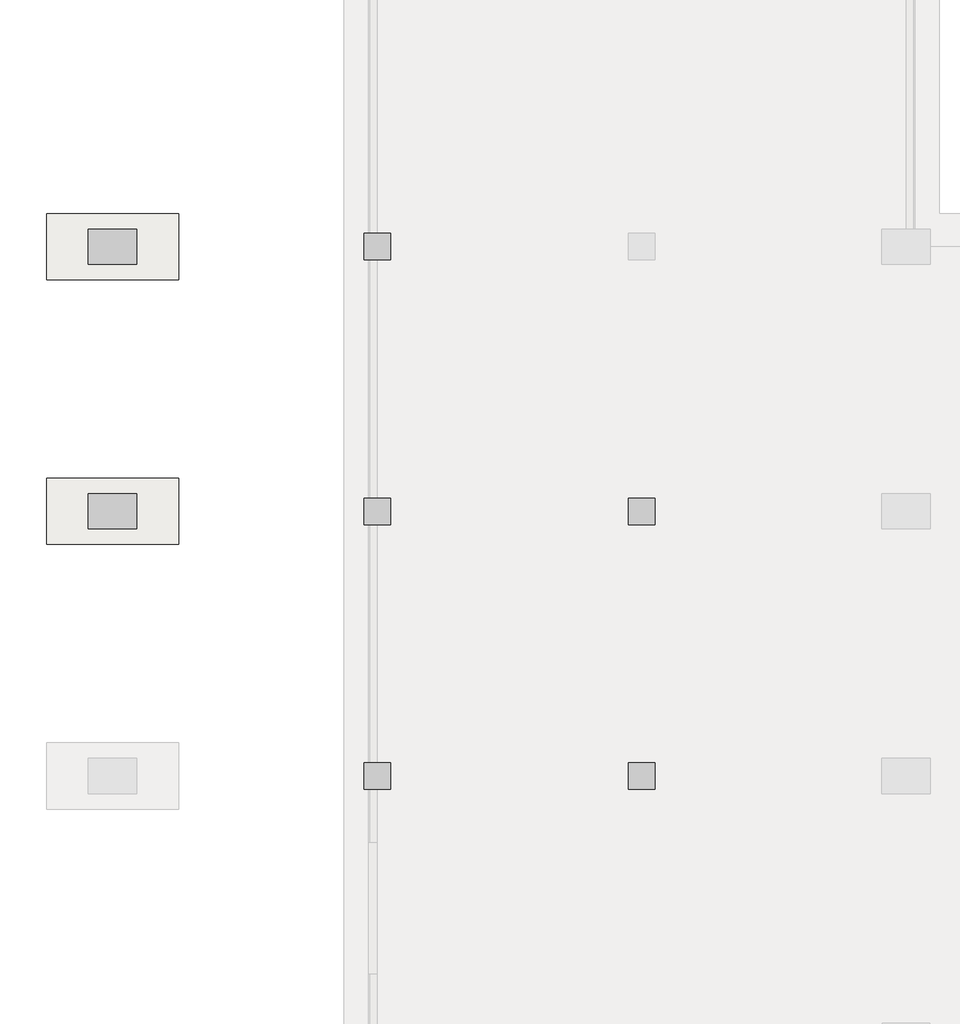
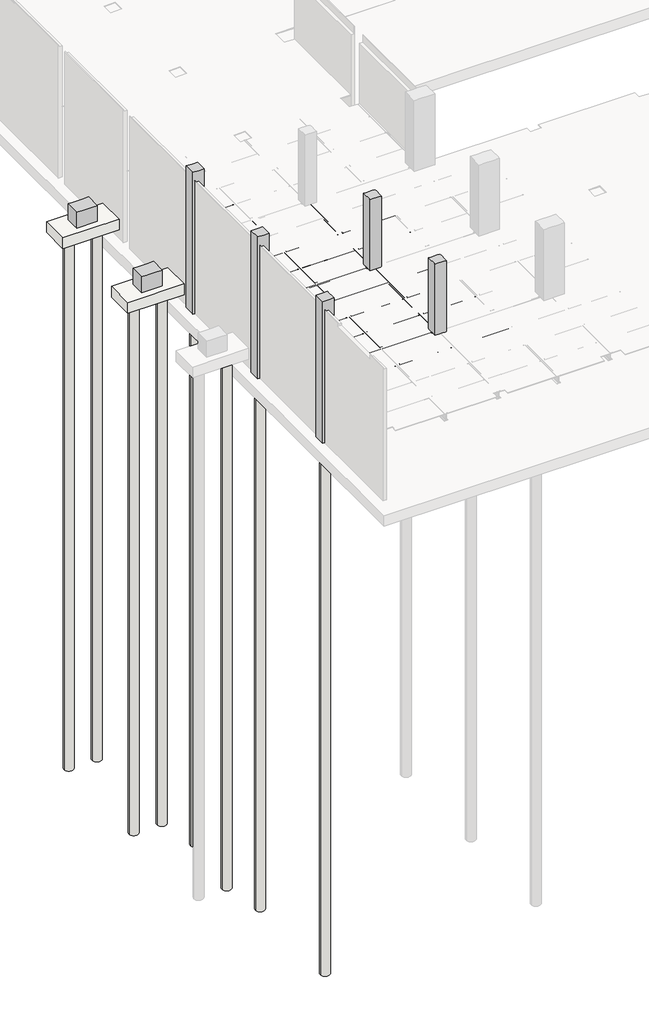
# Not in any storey, part 2 of 16: 26 beams, 10 slabs, 7 columns.
"""IFC4 building model written with IfcOpenShell, lengths in millimetres."""

from ifc_helpers import new_model, si_unit, point, frame, frame_2d, origin, place, context, project, spatial, polyline, circle_curve, trimmed, segment, composite_curve, outline, extrude, faceted_brep, element, save

model = new_model("IFC4")

# Units and contexts
model_context = context("Model", 3, world=origin())
ifc_project = project(units=[si_unit("LENGTHUNIT", "METRE", prefix="MILLI")], contexts=[model_context])

# Site, building
site = spatial("IfcSite", under=ifc_project)
building = spatial("IfcBuilding", under=site)

# Beams
placement = place(None, origin())
element("IfcBeam", 1, ObjectType="Steel Framing_H_KS : H_SB_AR_S02_H-400x200x8x13_BSG1", at=placement, inside=building, context=model_context, shape_type="SweptSolid", body=[
    extrude(outline(composite_curve([segment(polyline([(-47900.0, -4187.0381366), (-47900.0, -4200.0381366), (-48100.0, -4200.0381366), (-48100.0, -4187.0381366), (-48020.0, -4187.0381366)]), True, "CONTINUOUS"), segment(trimmed(circle_curve(frame_2d((-48020.0, -4171.0381366)), 16.0), [point((-48020.0, -4187.0381366))], [point((-48004.0, -4171.0381366))], True, "CARTESIAN"), True, "CONTINUOUS"), segment(polyline([(-48004.0, -4171.0381366), (-48004.0, -3829.0381366)]), True, "CONTINUOUS"), segment(trimmed(circle_curve(frame_2d((-48020.0, -3829.0381366)), 16.0), [point((-48004.0, -3829.0381366))], [point((-48020.0, -3813.0381366))], True, "CARTESIAN"), True, "CONTINUOUS"), segment(polyline([(-48020.0, -3813.0381366), (-48100.0, -3813.0381366), (-48100.0, -3800.0381366), (-47900.0, -3800.0381366), (-47900.0, -3813.0381366), (-47980.0, -3813.0381366)]), True, "CONTINUOUS"), segment(trimmed(circle_curve(frame_2d((-47980.0, -3829.0381366)), 16.0), [point((-47980.0, -3813.0381366))], [point((-47996.0, -3829.0381366))], True, "CARTESIAN"), True, "CONTINUOUS"), segment(polyline([(-47996.0, -3829.0381366), (-47996.0, -4171.0381366)]), True, "CONTINUOUS"), segment(trimmed(circle_curve(frame_2d((-47980.0, -4171.0381366)), 16.0), [point((-47996.0, -4171.0381366))], [point((-47980.0, -4187.0381366))], True, "CARTESIAN"), True, "CONTINUOUS"), segment(polyline([(-47980.0, -4187.0381366), (-47900.0, -4187.0381366)]), True, "CONTINUOUS")], self_intersect=False)), frame((24312.7, 0.0, 0.0), z_axis=(1.0, 0.0, 0.0), x_axis=(0.0, 1.0, 0.0)), (0.0, 0.0, 1.0), 5374.6),
])
element("IfcBeam", 2, ObjectType="Steel Framing_H_KS : H_SB_AR_S02_H-400x200x8x13_BSG2", at=placement, inside=building, context=model_context, shape_type="SweptSolid", body=[
    extrude(outline(composite_curve([segment(polyline([(-4187.0381366, 29900.0), (-4200.0381366, 29900.0), (-4200.0381366, 30100.0), (-4187.0381366, 30100.0), (-4187.0381366, 30020.0)]), True, "CONTINUOUS"), segment(trimmed(circle_curve(frame_2d((-4171.0381366, 30020.0)), 16.0), [point((-4187.0381366, 30020.0))], [point((-4171.0381366, 30004.0))], True, "CARTESIAN"), True, "CONTINUOUS"), segment(polyline([(-4171.0381366, 30004.0), (-3829.0381366, 30004.0)]), True, "CONTINUOUS"), segment(trimmed(circle_curve(frame_2d((-3829.0381366, 30020.0)), 16.0), [point((-3829.0381366, 30004.0))], [point((-3813.0381366, 30020.0))], True, "CARTESIAN"), True, "CONTINUOUS"), segment(polyline([(-3813.0381366, 30020.0), (-3813.0381366, 30100.0), (-3800.0381366, 30100.0), (-3800.0381366, 29900.0), (-3813.0381366, 29900.0), (-3813.0381366, 29980.0)]), True, "CONTINUOUS"), segment(trimmed(circle_curve(frame_2d((-3829.0381366, 29980.0)), 16.0), [point((-3813.0381366, 29980.0))], [point((-3829.0381366, 29996.0))], True, "CARTESIAN"), True, "CONTINUOUS"), segment(polyline([(-3829.0381366, 29996.0), (-4171.0381366, 29996.0)]), True, "CONTINUOUS"), segment(trimmed(circle_curve(frame_2d((-4171.0381366, 29980.0)), 16.0), [point((-4171.0381366, 29996.0))], [point((-4187.0381366, 29980.0))], True, "CARTESIAN"), True, "CONTINUOUS"), segment(polyline([(-4187.0381366, 29980.0), (-4187.0381366, 29900.0)]), True, "CONTINUOUS")], self_intersect=False)), frame((0.0, -47687.3, 0.0), z_axis=(0.0, 1.0, 0.0), x_axis=(0.0, 0.0, 1.0)), (0.0, 0.0, 1.0), 5374.6),
])
element("IfcBeam", 3, ObjectType="Steel Framing_H_KS : H_SB_AR_S02_H-400x200x8x13_BSB1", at=placement, inside=building, context=model_context, shape_type="SweptSolid", body=[
    extrude(outline(composite_curve([segment(polyline([(-4187.0381366, 26900.0), (-4200.0381366, 26900.0), (-4200.0381366, 27100.0), (-4187.0381366, 27100.0), (-4187.0381366, 27020.0)]), True, "CONTINUOUS"), segment(trimmed(circle_curve(frame_2d((-4171.0381366, 27020.0)), 16.0), [point((-4187.0381366, 27020.0))], [point((-4171.0381366, 27004.0))], True, "CARTESIAN"), True, "CONTINUOUS"), segment(polyline([(-4171.0381366, 27004.0), (-3829.0381366, 27004.0)]), True, "CONTINUOUS"), segment(trimmed(circle_curve(frame_2d((-3829.0381366, 27020.0)), 16.0), [point((-3829.0381366, 27004.0))], [point((-3813.0381366, 27020.0))], True, "CARTESIAN"), True, "CONTINUOUS"), segment(polyline([(-3813.0381366, 27020.0), (-3813.0381366, 27100.0), (-3800.0381366, 27100.0), (-3800.0381366, 26900.0), (-3813.0381366, 26900.0), (-3813.0381366, 26980.0)]), True, "CONTINUOUS"), segment(trimmed(circle_curve(frame_2d((-3829.0381366, 26980.0)), 16.0), [point((-3813.0381366, 26980.0))], [point((-3829.0381366, 26996.0))], True, "CARTESIAN"), True, "CONTINUOUS"), segment(polyline([(-3829.0381366, 26996.0), (-4171.0381366, 26996.0)]), True, "CONTINUOUS"), segment(trimmed(circle_curve(frame_2d((-4171.0381366, 26980.0)), 16.0), [point((-4171.0381366, 26996.0))], [point((-4187.0381366, 26980.0))], True, "CARTESIAN"), True, "CONTINUOUS"), segment(polyline([(-4187.0381366, 26980.0), (-4187.0381366, 26900.0)]), True, "CONTINUOUS")], self_intersect=False)), frame((0.0, -47887.3, 0.0), z_axis=(0.0, 1.0, 0.0), x_axis=(0.0, 0.0, 1.0)), (0.0, 0.0, 1.0), 5774.6),
])
element("IfcBeam", 4, ObjectType="Steel Framing_C_KS : H_SB_AR_S02_C-150x75x6.5x10_J1", at=placement, inside=building, context=model_context, shape_type="SweptSolid", body=[
    extrude(outline(composite_curve([segment(polyline([(-44977.2, -3800.0381366), (-44977.2, -3950.0381366), (-45052.2, -3950.0381366)]), True, "CONTINUOUS"), segment(trimmed(circle_curve(frame_2d((-45042.2, -3950.0381366)), 10.0), [point((-45052.2, -3950.0381366))], [point((-45042.2, -3940.0381366))], False, "CARTESIAN"), True, "CONTINUOUS"), segment(polyline([(-45042.2, -3940.0381366), (-44983.7, -3930.7726469), (-44983.7, -3819.3036264), (-45042.2, -3810.0381366)]), True, "CONTINUOUS"), segment(trimmed(circle_curve(frame_2d((-45042.2, -3800.0381366)), 10.0), [point((-45042.2, -3810.0381366))], [point((-45052.2, -3800.0381366))], False, "CARTESIAN"), True, "CONTINUOUS"), segment(polyline([(-45052.2, -3800.0381366), (-44977.2, -3800.0381366)]), True, "CONTINUOUS")], self_intersect=False)), frame((24000.0, 0.0, 0.0), z_axis=(1.0, 0.0, 0.0), x_axis=(0.0, 1.0, 0.0)), (0.0, 0.0, 1.0), 2887.3),
])
element("IfcBeam", 5, ObjectType="Steel Framing_C_KS : H_SB_AR_S02_C-150x75x6.5x10_J1", at=placement, inside=building, context=model_context, shape_type="SweptSolid", body=[
    extrude(outline(composite_curve([segment(polyline([(-46477.2, -3800.0381366), (-46477.2, -3950.0381366), (-46552.2, -3950.0381366)]), True, "CONTINUOUS"), segment(trimmed(circle_curve(frame_2d((-46542.2, -3950.0381366)), 10.0), [point((-46552.2, -3950.0381366))], [point((-46542.2, -3940.0381366))], False, "CARTESIAN"), True, "CONTINUOUS"), segment(polyline([(-46542.2, -3940.0381366), (-46483.7, -3930.7726469), (-46483.7, -3819.3036264), (-46542.2, -3810.0381366)]), True, "CONTINUOUS"), segment(trimmed(circle_curve(frame_2d((-46542.2, -3800.0381366)), 10.0), [point((-46542.2, -3810.0381366))], [point((-46552.2, -3800.0381366))], False, "CARTESIAN"), True, "CONTINUOUS"), segment(polyline([(-46552.2, -3800.0381366), (-46477.2, -3800.0381366)]), True, "CONTINUOUS")], self_intersect=False)), frame((24000.0, 0.0, 0.0), z_axis=(1.0, 0.0, 0.0), x_axis=(0.0, 1.0, 0.0)), (0.0, 0.0, 1.0), 2887.3),
])
element("IfcBeam", 6, ObjectType="Steel Framing_C_KS : H_SB_AR_S02_C-150x75x6.5x10_J1", at=placement, inside=building, context=model_context, shape_type="SweptSolid", body=[
    extrude(outline(composite_curve([segment(polyline([(-43477.2, -3800.0381366), (-43477.2, -3950.0381366), (-43552.2, -3950.0381366)]), True, "CONTINUOUS"), segment(trimmed(circle_curve(frame_2d((-43542.2, -3950.0381366)), 10.0), [point((-43552.2, -3950.0381366))], [point((-43542.2, -3940.0381366))], False, "CARTESIAN"), True, "CONTINUOUS"), segment(polyline([(-43542.2, -3940.0381366), (-43483.7, -3930.7726469), (-43483.7, -3819.3036264), (-43542.2, -3810.0381366)]), True, "CONTINUOUS"), segment(trimmed(circle_curve(frame_2d((-43542.2, -3800.0381366)), 10.0), [point((-43542.2, -3810.0381366))], [point((-43552.2, -3800.0381366))], False, "CARTESIAN"), True, "CONTINUOUS"), segment(polyline([(-43552.2, -3800.0381366), (-43477.2, -3800.0381366)]), True, "CONTINUOUS")], self_intersect=False)), frame((24000.0, 0.0, 0.0), z_axis=(1.0, 0.0, 0.0), x_axis=(0.0, 1.0, 0.0)), (0.0, 0.0, 1.0), 2887.3),
])
element("IfcBeam", 7, ObjectType="Steel Framing_C_KS : H_SB_AR_S02_C-150x75x6.5x10_J1", at=placement, inside=building, context=model_context, shape_type="SweptSolid", body=[
    extrude(outline(composite_curve([segment(polyline([(-44977.2, -3800.0381366), (-44977.2, -3950.0381366), (-45052.2, -3950.0381366)]), True, "CONTINUOUS"), segment(trimmed(circle_curve(frame_2d((-45042.2, -3950.0381366)), 10.0), [point((-45052.2, -3950.0381366))], [point((-45042.2, -3940.0381366))], False, "CARTESIAN"), True, "CONTINUOUS"), segment(polyline([(-45042.2, -3940.0381366), (-44983.7, -3930.7726469), (-44983.7, -3819.3036264), (-45042.2, -3810.0381366)]), True, "CONTINUOUS"), segment(trimmed(circle_curve(frame_2d((-45042.2, -3800.0381366)), 10.0), [point((-45042.2, -3810.0381366))], [point((-45052.2, -3800.0381366))], False, "CARTESIAN"), True, "CONTINUOUS"), segment(polyline([(-45052.2, -3800.0381366), (-44977.2, -3800.0381366)]), True, "CONTINUOUS")], self_intersect=False)), frame((27112.7, 0.0, 0.0), z_axis=(1.0, 0.0, 0.0), x_axis=(0.0, 1.0, 0.0)), (0.0, 0.0, 1.0), 2774.6),
])
element("IfcBeam", 8, ObjectType="Steel Framing_C_KS : H_SB_AR_S02_C-150x75x6.5x10_J1", at=placement, inside=building, context=model_context, shape_type="SweptSolid", body=[
    extrude(outline(composite_curve([segment(polyline([(-46477.2, -3800.0381366), (-46477.2, -3950.0381366), (-46552.2, -3950.0381366)]), True, "CONTINUOUS"), segment(trimmed(circle_curve(frame_2d((-46542.2, -3950.0381366)), 10.0), [point((-46552.2, -3950.0381366))], [point((-46542.2, -3940.0381366))], False, "CARTESIAN"), True, "CONTINUOUS"), segment(polyline([(-46542.2, -3940.0381366), (-46483.7, -3930.7726469), (-46483.7, -3819.3036264), (-46542.2, -3810.0381366)]), True, "CONTINUOUS"), segment(trimmed(circle_curve(frame_2d((-46542.2, -3800.0381366)), 10.0), [point((-46542.2, -3810.0381366))], [point((-46552.2, -3800.0381366))], False, "CARTESIAN"), True, "CONTINUOUS"), segment(polyline([(-46552.2, -3800.0381366), (-46477.2, -3800.0381366)]), True, "CONTINUOUS")], self_intersect=False)), frame((27112.7, 0.0, 0.0), z_axis=(1.0, 0.0, 0.0), x_axis=(0.0, 1.0, 0.0)), (0.0, 0.0, 1.0), 2774.6),
])
element("IfcBeam", 9, ObjectType="Steel Framing_C_KS : H_SB_AR_S02_C-150x75x6.5x10_J1", at=placement, inside=building, context=model_context, shape_type="SweptSolid", body=[
    extrude(outline(composite_curve([segment(polyline([(-44977.2, -3800.0381366), (-44977.2, -3950.0381366), (-45052.2, -3950.0381366)]), True, "CONTINUOUS"), segment(trimmed(circle_curve(frame_2d((-45042.2, -3950.0381366)), 10.0), [point((-45052.2, -3950.0381366))], [point((-45042.2, -3940.0381366))], False, "CARTESIAN"), True, "CONTINUOUS"), segment(polyline([(-45042.2, -3940.0381366), (-44983.7, -3930.7726469), (-44983.7, -3819.3036264), (-45042.2, -3810.0381366)]), True, "CONTINUOUS"), segment(trimmed(circle_curve(frame_2d((-45042.2, -3800.0381366)), 10.0), [point((-45042.2, -3810.0381366))], [point((-45052.2, -3800.0381366))], False, "CARTESIAN"), True, "CONTINUOUS"), segment(polyline([(-45052.2, -3800.0381366), (-44977.2, -3800.0381366)]), True, "CONTINUOUS")], self_intersect=False)), frame((30112.7, 0.0, 0.0), z_axis=(1.0, 0.0, 0.0), x_axis=(0.0, 1.0, 0.0)), (0.0, 0.0, 1.0), 2774.6),
])
element("IfcBeam", 10, ObjectType="Steel Framing_C_KS : H_SB_AR_S02_C-150x75x6.5x10_J1", at=placement, inside=building, context=model_context, shape_type="SweptSolid", body=[
    extrude(outline(composite_curve([segment(polyline([(-46477.2, -3800.0381366), (-46477.2, -3950.0381366), (-46552.2, -3950.0381366)]), True, "CONTINUOUS"), segment(trimmed(circle_curve(frame_2d((-46542.2, -3950.0381366)), 10.0), [point((-46552.2, -3950.0381366))], [point((-46542.2, -3940.0381366))], False, "CARTESIAN"), True, "CONTINUOUS"), segment(polyline([(-46542.2, -3940.0381366), (-46483.7, -3930.7726469), (-46483.7, -3819.3036264), (-46542.2, -3810.0381366)]), True, "CONTINUOUS"), segment(trimmed(circle_curve(frame_2d((-46542.2, -3800.0381366)), 10.0), [point((-46542.2, -3810.0381366))], [point((-46552.2, -3800.0381366))], False, "CARTESIAN"), True, "CONTINUOUS"), segment(polyline([(-46552.2, -3800.0381366), (-46477.2, -3800.0381366)]), True, "CONTINUOUS")], self_intersect=False)), frame((30112.7, 0.0, 0.0), z_axis=(1.0, 0.0, 0.0), x_axis=(0.0, 1.0, 0.0)), (0.0, 0.0, 1.0), 2774.6),
])
element("IfcBeam", 11, ObjectType="Steel Framing_H_KS : H_SB_AR_S02_H-400x200x8x13_BSG1", at=placement, inside=building, context=model_context, shape_type="SweptSolid", body=[
    extrude(outline(composite_curve([segment(polyline([(-53900.0, -4187.0381366), (-53900.0, -4200.0381366), (-54100.0, -4200.0381366), (-54100.0, -4187.0381366), (-54020.0, -4187.0381366)]), True, "CONTINUOUS"), segment(trimmed(circle_curve(frame_2d((-54020.0, -4171.0381366)), 16.0), [point((-54020.0, -4187.0381366))], [point((-54004.0, -4171.0381366))], True, "CARTESIAN"), True, "CONTINUOUS"), segment(polyline([(-54004.0, -4171.0381366), (-54004.0, -3829.0381366)]), True, "CONTINUOUS"), segment(trimmed(circle_curve(frame_2d((-54020.0, -3829.0381366)), 16.0), [point((-54004.0, -3829.0381366))], [point((-54020.0, -3813.0381366))], True, "CARTESIAN"), True, "CONTINUOUS"), segment(polyline([(-54020.0, -3813.0381366), (-54100.0, -3813.0381366), (-54100.0, -3800.0381366), (-53900.0, -3800.0381366), (-53900.0, -3813.0381366), (-53980.0, -3813.0381366)]), True, "CONTINUOUS"), segment(trimmed(circle_curve(frame_2d((-53980.0, -3829.0381366)), 16.0), [point((-53980.0, -3813.0381366))], [point((-53996.0, -3829.0381366))], True, "CARTESIAN"), True, "CONTINUOUS"), segment(polyline([(-53996.0, -3829.0381366), (-53996.0, -4171.0381366)]), True, "CONTINUOUS"), segment(trimmed(circle_curve(frame_2d((-53980.0, -4171.0381366)), 16.0), [point((-53996.0, -4171.0381366))], [point((-53980.0, -4187.0381366))], True, "CARTESIAN"), True, "CONTINUOUS"), segment(polyline([(-53980.0, -4187.0381366), (-53900.0, -4187.0381366)]), True, "CONTINUOUS")], self_intersect=False)), frame((24312.7, 0.0, 0.0), z_axis=(1.0, 0.0, 0.0), x_axis=(0.0, 1.0, 0.0)), (0.0, 0.0, 1.0), 5374.6),
])
element("IfcBeam", 12, ObjectType="Steel Framing_H_KS : H_SB_AR_S02_H-400x200x8x13_BSG2", at=placement, inside=building, context=model_context, shape_type="SweptSolid", body=[
    extrude(outline(composite_curve([segment(polyline([(-4187.0381366, 29900.0), (-4200.0381366, 29900.0), (-4200.0381366, 30100.0), (-4187.0381366, 30100.0), (-4187.0381366, 30020.0)]), True, "CONTINUOUS"), segment(trimmed(circle_curve(frame_2d((-4171.0381366, 30020.0)), 16.0), [point((-4187.0381366, 30020.0))], [point((-4171.0381366, 30004.0))], True, "CARTESIAN"), True, "CONTINUOUS"), segment(polyline([(-4171.0381366, 30004.0), (-3829.0381366, 30004.0)]), True, "CONTINUOUS"), segment(trimmed(circle_curve(frame_2d((-3829.0381366, 30020.0)), 16.0), [point((-3829.0381366, 30004.0))], [point((-3813.0381366, 30020.0))], True, "CARTESIAN"), True, "CONTINUOUS"), segment(polyline([(-3813.0381366, 30020.0), (-3813.0381366, 30100.0), (-3800.0381366, 30100.0), (-3800.0381366, 29900.0), (-3813.0381366, 29900.0), (-3813.0381366, 29980.0)]), True, "CONTINUOUS"), segment(trimmed(circle_curve(frame_2d((-3829.0381366, 29980.0)), 16.0), [point((-3813.0381366, 29980.0))], [point((-3829.0381366, 29996.0))], True, "CARTESIAN"), True, "CONTINUOUS"), segment(polyline([(-3829.0381366, 29996.0), (-4171.0381366, 29996.0)]), True, "CONTINUOUS"), segment(trimmed(circle_curve(frame_2d((-4171.0381366, 29980.0)), 16.0), [point((-4171.0381366, 29996.0))], [point((-4187.0381366, 29980.0))], True, "CARTESIAN"), True, "CONTINUOUS"), segment(polyline([(-4187.0381366, 29980.0), (-4187.0381366, 29900.0)]), True, "CONTINUOUS")], self_intersect=False)), frame((0.0, -53687.3, 0.0), z_axis=(0.0, 1.0, 0.0), x_axis=(0.0, 0.0, 1.0)), (0.0, 0.0, 1.0), 5374.6),
])
element("IfcBeam", 13, ObjectType="Steel Framing_H_KS : H_SB_AR_S02_H-400x200x8x13_BSB1", at=placement, inside=building, context=model_context, shape_type="SweptSolid", body=[
    extrude(outline(composite_curve([segment(polyline([(-4187.0381366, 26900.0), (-4200.0381366, 26900.0), (-4200.0381366, 27100.0), (-4187.0381366, 27100.0), (-4187.0381366, 27020.0)]), True, "CONTINUOUS"), segment(trimmed(circle_curve(frame_2d((-4171.0381366, 27020.0)), 16.0), [point((-4187.0381366, 27020.0))], [point((-4171.0381366, 27004.0))], True, "CARTESIAN"), True, "CONTINUOUS"), segment(polyline([(-4171.0381366, 27004.0), (-3829.0381366, 27004.0)]), True, "CONTINUOUS"), segment(trimmed(circle_curve(frame_2d((-3829.0381366, 27020.0)), 16.0), [point((-3829.0381366, 27004.0))], [point((-3813.0381366, 27020.0))], True, "CARTESIAN"), True, "CONTINUOUS"), segment(polyline([(-3813.0381366, 27020.0), (-3813.0381366, 27100.0), (-3800.0381366, 27100.0), (-3800.0381366, 26900.0), (-3813.0381366, 26900.0), (-3813.0381366, 26980.0)]), True, "CONTINUOUS"), segment(trimmed(circle_curve(frame_2d((-3829.0381366, 26980.0)), 16.0), [point((-3813.0381366, 26980.0))], [point((-3829.0381366, 26996.0))], True, "CARTESIAN"), True, "CONTINUOUS"), segment(polyline([(-3829.0381366, 26996.0), (-4171.0381366, 26996.0)]), True, "CONTINUOUS"), segment(trimmed(circle_curve(frame_2d((-4171.0381366, 26980.0)), 16.0), [point((-4171.0381366, 26996.0))], [point((-4187.0381366, 26980.0))], True, "CARTESIAN"), True, "CONTINUOUS"), segment(polyline([(-4187.0381366, 26980.0), (-4187.0381366, 26900.0)]), True, "CONTINUOUS")], self_intersect=False)), frame((0.0, -53887.3, 0.0), z_axis=(0.0, 1.0, 0.0), x_axis=(0.0, 0.0, 1.0)), (0.0, 0.0, 1.0), 5774.6),
])
element("IfcBeam", 14, ObjectType="Steel Framing_C_KS : H_SB_AR_S02_C-150x75x6.5x10_J1", at=placement, inside=building, context=model_context, shape_type="SweptSolid", body=[
    extrude(outline(composite_curve([segment(polyline([(-50977.2, -3800.0381366), (-50977.2, -3950.0381366), (-51052.2, -3950.0381366)]), True, "CONTINUOUS"), segment(trimmed(circle_curve(frame_2d((-51042.2, -3950.0381366)), 10.0), [point((-51052.2, -3950.0381366))], [point((-51042.2, -3940.0381366))], False, "CARTESIAN"), True, "CONTINUOUS"), segment(polyline([(-51042.2, -3940.0381366), (-50983.7, -3930.7726469), (-50983.7, -3819.3036264), (-51042.2, -3810.0381366)]), True, "CONTINUOUS"), segment(trimmed(circle_curve(frame_2d((-51042.2, -3800.0381366)), 10.0), [point((-51042.2, -3810.0381366))], [point((-51052.2, -3800.0381366))], False, "CARTESIAN"), True, "CONTINUOUS"), segment(polyline([(-51052.2, -3800.0381366), (-50977.2, -3800.0381366)]), True, "CONTINUOUS")], self_intersect=False)), frame((24000.0, 0.0, 0.0), z_axis=(1.0, 0.0, 0.0), x_axis=(0.0, 1.0, 0.0)), (0.0, 0.0, 1.0), 2887.3),
])
element("IfcBeam", 15, ObjectType="Steel Framing_C_KS : H_SB_AR_S02_C-150x75x6.5x10_J1", at=placement, inside=building, context=model_context, shape_type="SweptSolid", body=[
    extrude(outline(composite_curve([segment(polyline([(-52477.2, -3800.0381366), (-52477.2, -3950.0381366), (-52552.2, -3950.0381366)]), True, "CONTINUOUS"), segment(trimmed(circle_curve(frame_2d((-52542.2, -3950.0381366)), 10.0), [point((-52552.2, -3950.0381366))], [point((-52542.2, -3940.0381366))], False, "CARTESIAN"), True, "CONTINUOUS"), segment(polyline([(-52542.2, -3940.0381366), (-52483.7, -3930.7726469), (-52483.7, -3819.3036264), (-52542.2, -3810.0381366)]), True, "CONTINUOUS"), segment(trimmed(circle_curve(frame_2d((-52542.2, -3800.0381366)), 10.0), [point((-52542.2, -3810.0381366))], [point((-52552.2, -3800.0381366))], False, "CARTESIAN"), True, "CONTINUOUS"), segment(polyline([(-52552.2, -3800.0381366), (-52477.2, -3800.0381366)]), True, "CONTINUOUS")], self_intersect=False)), frame((24000.0, 0.0, 0.0), z_axis=(1.0, 0.0, 0.0), x_axis=(0.0, 1.0, 0.0)), (0.0, 0.0, 1.0), 2887.3),
])
element("IfcBeam", 16, ObjectType="Steel Framing_C_KS : H_SB_AR_S02_C-150x75x6.5x10_J1", at=placement, inside=building, context=model_context, shape_type="SweptSolid", body=[
    extrude(outline(composite_curve([segment(polyline([(-49477.2, -3800.0381366), (-49477.2, -3950.0381366), (-49552.2, -3950.0381366)]), True, "CONTINUOUS"), segment(trimmed(circle_curve(frame_2d((-49542.2, -3950.0381366)), 10.0), [point((-49552.2, -3950.0381366))], [point((-49542.2, -3940.0381366))], False, "CARTESIAN"), True, "CONTINUOUS"), segment(polyline([(-49542.2, -3940.0381366), (-49483.7, -3930.7726469), (-49483.7, -3819.3036264), (-49542.2, -3810.0381366)]), True, "CONTINUOUS"), segment(trimmed(circle_curve(frame_2d((-49542.2, -3800.0381366)), 10.0), [point((-49542.2, -3810.0381366))], [point((-49552.2, -3800.0381366))], False, "CARTESIAN"), True, "CONTINUOUS"), segment(polyline([(-49552.2, -3800.0381366), (-49477.2, -3800.0381366)]), True, "CONTINUOUS")], self_intersect=False)), frame((24000.0, 0.0, 0.0), z_axis=(1.0, 0.0, 0.0), x_axis=(0.0, 1.0, 0.0)), (0.0, 0.0, 1.0), 2887.3),
])
element("IfcBeam", 17, ObjectType="Steel Framing_C_KS : H_SB_AR_S02_C-150x75x6.5x10_J1", at=placement, inside=building, context=model_context, shape_type="SweptSolid", body=[
    extrude(outline(composite_curve([segment(polyline([(-50977.2, -3800.0381366), (-50977.2, -3950.0381366), (-51052.2, -3950.0381366)]), True, "CONTINUOUS"), segment(trimmed(circle_curve(frame_2d((-51042.2, -3950.0381366)), 10.0), [point((-51052.2, -3950.0381366))], [point((-51042.2, -3940.0381366))], False, "CARTESIAN"), True, "CONTINUOUS"), segment(polyline([(-51042.2, -3940.0381366), (-50983.7, -3930.7726469), (-50983.7, -3819.3036264), (-51042.2, -3810.0381366)]), True, "CONTINUOUS"), segment(trimmed(circle_curve(frame_2d((-51042.2, -3800.0381366)), 10.0), [point((-51042.2, -3810.0381366))], [point((-51052.2, -3800.0381366))], False, "CARTESIAN"), True, "CONTINUOUS"), segment(polyline([(-51052.2, -3800.0381366), (-50977.2, -3800.0381366)]), True, "CONTINUOUS")], self_intersect=False)), frame((27112.7, 0.0, 0.0), z_axis=(1.0, 0.0, 0.0), x_axis=(0.0, 1.0, 0.0)), (0.0, 0.0, 1.0), 2774.6),
])
element("IfcBeam", 18, ObjectType="Steel Framing_C_KS : H_SB_AR_S02_C-150x75x6.5x10_J1", at=placement, inside=building, context=model_context, shape_type="SweptSolid", body=[
    extrude(outline(composite_curve([segment(polyline([(-52477.2, -3800.0381366), (-52477.2, -3950.0381366), (-52552.2, -3950.0381366)]), True, "CONTINUOUS"), segment(trimmed(circle_curve(frame_2d((-52542.2, -3950.0381366)), 10.0), [point((-52552.2, -3950.0381366))], [point((-52542.2, -3940.0381366))], False, "CARTESIAN"), True, "CONTINUOUS"), segment(polyline([(-52542.2, -3940.0381366), (-52483.7, -3930.7726469), (-52483.7, -3819.3036264), (-52542.2, -3810.0381366)]), True, "CONTINUOUS"), segment(trimmed(circle_curve(frame_2d((-52542.2, -3800.0381366)), 10.0), [point((-52542.2, -3810.0381366))], [point((-52552.2, -3800.0381366))], False, "CARTESIAN"), True, "CONTINUOUS"), segment(polyline([(-52552.2, -3800.0381366), (-52477.2, -3800.0381366)]), True, "CONTINUOUS")], self_intersect=False)), frame((27112.7, 0.0, 0.0), z_axis=(1.0, 0.0, 0.0), x_axis=(0.0, 1.0, 0.0)), (0.0, 0.0, 1.0), 2774.6),
])
element("IfcBeam", 19, ObjectType="Steel Framing_C_KS : H_SB_AR_S02_C-150x75x6.5x10_J1", at=placement, inside=building, context=model_context, shape_type="SweptSolid", body=[
    extrude(outline(composite_curve([segment(polyline([(-49477.2, -3800.0381366), (-49477.2, -3950.0381366), (-49552.2, -3950.0381366)]), True, "CONTINUOUS"), segment(trimmed(circle_curve(frame_2d((-49542.2, -3950.0381366)), 10.0), [point((-49552.2, -3950.0381366))], [point((-49542.2, -3940.0381366))], False, "CARTESIAN"), True, "CONTINUOUS"), segment(polyline([(-49542.2, -3940.0381366), (-49483.7, -3930.7726469), (-49483.7, -3819.3036264), (-49542.2, -3810.0381366)]), True, "CONTINUOUS"), segment(trimmed(circle_curve(frame_2d((-49542.2, -3800.0381366)), 10.0), [point((-49542.2, -3810.0381366))], [point((-49552.2, -3800.0381366))], False, "CARTESIAN"), True, "CONTINUOUS"), segment(polyline([(-49552.2, -3800.0381366), (-49477.2, -3800.0381366)]), True, "CONTINUOUS")], self_intersect=False)), frame((27112.7, 0.0, 0.0), z_axis=(1.0, 0.0, 0.0), x_axis=(0.0, 1.0, 0.0)), (0.0, 0.0, 1.0), 2774.6),
])
element("IfcBeam", 20, ObjectType="Steel Framing_C_KS : H_SB_AR_S02_C-150x75x6.5x10_J1", at=placement, inside=building, context=model_context, shape_type="SweptSolid", body=[
    extrude(outline(composite_curve([segment(polyline([(-50977.2, -3800.0381366), (-50977.2, -3950.0381366), (-51052.2, -3950.0381366)]), True, "CONTINUOUS"), segment(trimmed(circle_curve(frame_2d((-51042.2, -3950.0381366)), 10.0), [point((-51052.2, -3950.0381366))], [point((-51042.2, -3940.0381366))], False, "CARTESIAN"), True, "CONTINUOUS"), segment(polyline([(-51042.2, -3940.0381366), (-50983.7, -3930.7726469), (-50983.7, -3819.3036264), (-51042.2, -3810.0381366)]), True, "CONTINUOUS"), segment(trimmed(circle_curve(frame_2d((-51042.2, -3800.0381366)), 10.0), [point((-51042.2, -3810.0381366))], [point((-51052.2, -3800.0381366))], False, "CARTESIAN"), True, "CONTINUOUS"), segment(polyline([(-51052.2, -3800.0381366), (-50977.2, -3800.0381366)]), True, "CONTINUOUS")], self_intersect=False)), frame((30112.7, 0.0, 0.0), z_axis=(1.0, 0.0, 0.0), x_axis=(0.0, 1.0, 0.0)), (0.0, 0.0, 1.0), 2774.6),
])
element("IfcBeam", 21, ObjectType="Steel Framing_C_KS : H_SB_AR_S02_C-150x75x6.5x10_J1", at=placement, inside=building, context=model_context, shape_type="SweptSolid", body=[
    extrude(outline(composite_curve([segment(polyline([(-52477.2, -3800.0381366), (-52477.2, -3950.0381366), (-52552.2, -3950.0381366)]), True, "CONTINUOUS"), segment(trimmed(circle_curve(frame_2d((-52542.2, -3950.0381366)), 10.0), [point((-52552.2, -3950.0381366))], [point((-52542.2, -3940.0381366))], False, "CARTESIAN"), True, "CONTINUOUS"), segment(polyline([(-52542.2, -3940.0381366), (-52483.7, -3930.7726469), (-52483.7, -3819.3036264), (-52542.2, -3810.0381366)]), True, "CONTINUOUS"), segment(trimmed(circle_curve(frame_2d((-52542.2, -3800.0381366)), 10.0), [point((-52542.2, -3810.0381366))], [point((-52552.2, -3800.0381366))], False, "CARTESIAN"), True, "CONTINUOUS"), segment(polyline([(-52552.2, -3800.0381366), (-52477.2, -3800.0381366)]), True, "CONTINUOUS")], self_intersect=False)), frame((30112.7, 0.0, 0.0), z_axis=(1.0, 0.0, 0.0), x_axis=(0.0, 1.0, 0.0)), (0.0, 0.0, 1.0), 2774.6),
])
element("IfcBeam", 22, ObjectType="Steel Framing_C_KS : H_SB_AR_S02_C-150x75x6.5x10_J1", at=placement, inside=building, context=model_context, shape_type="SweptSolid", body=[
    extrude(outline(composite_curve([segment(polyline([(-49477.2, -3800.0381366), (-49477.2, -3950.0381366), (-49552.2, -3950.0381366)]), True, "CONTINUOUS"), segment(trimmed(circle_curve(frame_2d((-49542.2, -3950.0381366)), 10.0), [point((-49552.2, -3950.0381366))], [point((-49542.2, -3940.0381366))], False, "CARTESIAN"), True, "CONTINUOUS"), segment(polyline([(-49542.2, -3940.0381366), (-49483.7, -3930.7726469), (-49483.7, -3819.3036264), (-49542.2, -3810.0381366)]), True, "CONTINUOUS"), segment(trimmed(circle_curve(frame_2d((-49542.2, -3800.0381366)), 10.0), [point((-49542.2, -3810.0381366))], [point((-49552.2, -3800.0381366))], False, "CARTESIAN"), True, "CONTINUOUS"), segment(polyline([(-49552.2, -3800.0381366), (-49477.2, -3800.0381366)]), True, "CONTINUOUS")], self_intersect=False)), frame((30112.7, 0.0, 0.0), z_axis=(1.0, 0.0, 0.0), x_axis=(0.0, 1.0, 0.0)), (0.0, 0.0, 1.0), 2774.6),
])
element("IfcBeam", 23, ObjectType="Steel Framing_C_KS : H_SB_AR_S02_C-150x75x6.5x10_J1", at=placement, inside=building, context=model_context, shape_type="SweptSolid", body=[
    extrude(outline(composite_curve([segment(polyline([(-55477.2, -3800.0381366), (-55477.2, -3950.0381366), (-55552.2, -3950.0381366)]), True, "CONTINUOUS"), segment(trimmed(circle_curve(frame_2d((-55542.2, -3950.0381366)), 10.0), [point((-55552.2, -3950.0381366))], [point((-55542.2, -3940.0381366))], False, "CARTESIAN"), True, "CONTINUOUS"), segment(polyline([(-55542.2, -3940.0381366), (-55483.7, -3930.7726469), (-55483.7, -3819.3036264), (-55542.2, -3810.0381366)]), True, "CONTINUOUS"), segment(trimmed(circle_curve(frame_2d((-55542.2, -3800.0381366)), 10.0), [point((-55542.2, -3810.0381366))], [point((-55552.2, -3800.0381366))], False, "CARTESIAN"), True, "CONTINUOUS"), segment(polyline([(-55552.2, -3800.0381366), (-55477.2, -3800.0381366)]), True, "CONTINUOUS")], self_intersect=False)), frame((24000.0, 0.0, 0.0), z_axis=(1.0, 0.0, 0.0), x_axis=(0.0, 1.0, 0.0)), (0.0, 0.0, 1.0), 2887.3),
])
element("IfcBeam", 24, ObjectType="Steel Framing_C_KS : H_SB_AR_S02_C-150x75x6.5x10_J1", at=placement, inside=building, context=model_context, shape_type="SweptSolid", body=[
    extrude(outline(composite_curve([segment(polyline([(-55477.2, -3800.0381366), (-55477.2, -3950.0381366), (-55552.2, -3950.0381366)]), True, "CONTINUOUS"), segment(trimmed(circle_curve(frame_2d((-55542.2, -3950.0381366)), 10.0), [point((-55552.2, -3950.0381366))], [point((-55542.2, -3940.0381366))], False, "CARTESIAN"), True, "CONTINUOUS"), segment(polyline([(-55542.2, -3940.0381366), (-55483.7, -3930.7726469), (-55483.7, -3819.3036264), (-55542.2, -3810.0381366)]), True, "CONTINUOUS"), segment(trimmed(circle_curve(frame_2d((-55542.2, -3800.0381366)), 10.0), [point((-55542.2, -3810.0381366))], [point((-55552.2, -3800.0381366))], False, "CARTESIAN"), True, "CONTINUOUS"), segment(polyline([(-55552.2, -3800.0381366), (-55477.2, -3800.0381366)]), True, "CONTINUOUS")], self_intersect=False)), frame((27112.7, 0.0, 0.0), z_axis=(1.0, 0.0, 0.0), x_axis=(0.0, 1.0, 0.0)), (0.0, 0.0, 1.0), 2774.6),
])
element("IfcBeam", 25, ObjectType="Steel Framing_C_KS : H_SB_AR_S02_C-150x75x6.5x10_J1", at=placement, inside=building, context=model_context, shape_type="SweptSolid", body=[
    extrude(outline(composite_curve([segment(polyline([(-55477.2, -3800.0381366), (-55477.2, -3950.0381366), (-55552.2, -3950.0381366)]), True, "CONTINUOUS"), segment(trimmed(circle_curve(frame_2d((-55542.2, -3950.0381366)), 10.0), [point((-55552.2, -3950.0381366))], [point((-55542.2, -3940.0381366))], False, "CARTESIAN"), True, "CONTINUOUS"), segment(polyline([(-55542.2, -3940.0381366), (-55483.7, -3930.7726469), (-55483.7, -3819.3036264), (-55542.2, -3810.0381366)]), True, "CONTINUOUS"), segment(trimmed(circle_curve(frame_2d((-55542.2, -3800.0381366)), 10.0), [point((-55542.2, -3810.0381366))], [point((-55552.2, -3800.0381366))], False, "CARTESIAN"), True, "CONTINUOUS"), segment(polyline([(-55552.2, -3800.0381366), (-55477.2, -3800.0381366)]), True, "CONTINUOUS")], self_intersect=False)), frame((30112.7, 0.0, 0.0), z_axis=(1.0, 0.0, 0.0), x_axis=(0.0, 1.0, 0.0)), (0.0, 0.0, 1.0), 2774.6),
])
element("IfcBeam", 26, ObjectType="Steel Framing_C_KS : H_SB_AR_S02_C-150x75x6.5x10_J1", at=placement, inside=building, context=model_context, shape_type="SweptSolid", body=[
    extrude(outline(composite_curve([segment(polyline([(-40477.2, -3800.0381366), (-40477.2, -3950.0381366), (-40552.2, -3950.0381366)]), True, "CONTINUOUS"), segment(trimmed(circle_curve(frame_2d((-40542.2, -3950.0381366)), 10.0), [point((-40552.2, -3950.0381366))], [point((-40542.2, -3940.0381366))], False, "CARTESIAN"), True, "CONTINUOUS"), segment(polyline([(-40542.2, -3940.0381366), (-40483.7, -3930.7726469), (-40483.7, -3819.3036264), (-40542.2, -3810.0381366)]), True, "CONTINUOUS"), segment(trimmed(circle_curve(frame_2d((-40542.2, -3800.0381366)), 10.0), [point((-40542.2, -3810.0381366))], [point((-40552.2, -3800.0381366))], False, "CARTESIAN"), True, "CONTINUOUS"), segment(polyline([(-40552.2, -3800.0381366), (-40477.2, -3800.0381366)]), True, "CONTINUOUS")], self_intersect=False)), frame((24000.0, 0.0, 0.0), z_axis=(1.0, 0.0, 0.0), x_axis=(0.0, 1.0, 0.0)), (0.0, 0.0, 1.0), 2887.3),
])

# Columns
element("IfcColumn", 27, ObjectType="RC_Column_Rectangular : H_SC_AR_S15_UG PED_Bit_800x1100_PD1", at=placement, inside=building, context=model_context, shape_type="Brep", body=[
    faceted_brep([(17450.0, -41600.0, -700.0381366), (18550.0, -41600.0, -700.0381366), (18550.0, -42400.0, -700.0381366), (17450.0, -42400.0, -700.0381366), (17450.0, -41600.0, 199.9618634), (17800.0, -41600.0, 199.9618634), (18200.0, -41600.0, 199.9618634), (18550.0, -41600.0, 199.9618634), (18550.0, -41600.0, -0.0381366), (18550.0, -42400.0, 199.9618634), (18550.0, -42400.0, -0.0381366), (18200.0, -42400.0, 199.9618634), (17800.0, -42400.0, 199.9618634), (17450.0, -42400.0, 199.9618634)], [[[0, 1, 2, 3]], [[4, 5, 6, 7, 8, 1, 0]], [[7, 9, 10, 2, 1, 8]], [[9, 11, 12, 13, 3, 2, 10]], [[13, 4, 0, 3]], [[4, 13, 12, 11, 9, 7, 6, 5]]]),
])
element("IfcColumn", 28, ObjectType="RC_Column_Rectangular : H_SC_AR_S15_UG PED_Bit_800x1100_PD1", at=placement, inside=building, context=model_context, shape_type="Brep", body=[
    faceted_brep([(17450.0, -47600.0, -700.0381366), (18550.0, -47600.0, -700.0381366), (18550.0, -48400.0, -700.0381366), (17450.0, -48400.0, -700.0381366), (17450.0, -47600.0, 199.9618634), (17800.0, -47600.0, 199.9618634), (18200.0, -47600.0, 199.9618634), (18550.0, -47600.0, 199.9618634), (18550.0, -47600.0, -0.0381366), (18550.0, -48400.0, 199.9618634), (18550.0, -48400.0, -0.0381366), (18200.0, -48400.0, 199.9618634), (17800.0, -48400.0, 199.9618634), (17450.0, -48400.0, 199.9618634)], [[[0, 1, 2, 3]], [[4, 5, 6, 7, 8, 1, 0]], [[7, 9, 10, 2, 1, 8]], [[9, 11, 12, 13, 3, 2, 10]], [[13, 4, 0, 3]], [[4, 13, 12, 11, 9, 7, 6, 5]]]),
])
element("IfcColumn", 29, ObjectType="RC_Column_Rectangular : H_SC_AR_S15_UG PED_Bit_600x600_BC1", at=placement, inside=building, context=model_context, shape_type="Brep", body=[
    faceted_brep([(24300.0, -41700.0, -7800.0381366), (24300.0, -42300.0, -7800.0381366), (24000.0, -42300.0, -7800.0381366), (23800.0, -42300.0, -7800.0381366), (23700.0, -42300.0, -7800.0381366), (23700.0, -41700.0, -7800.0381366), (23800.0, -41700.0, -7800.0381366), (24000.0, -41700.0, -7800.0381366), (24300.0, -41700.0, 199.9618634), (24300.0, -41825.0, 199.9618634), (24300.0, -42175.0, 199.9618634), (24300.0, -42300.0, 199.9618634), (24300.0, -42300.0, -0.0381366), (24300.0, -42300.0, -3800.0381366), (24300.0, -42300.0, -3832.0381366), (24300.0, -41700.0, -3832.0381366), (24300.0, -41700.0, -3800.0381366), (24300.0, -41700.0, -0.0381366), (24000.0, -42300.0, 199.9618634), (23700.0, -42300.0, 199.9618634), (23700.0, -42300.0, -0.0381366), (23700.0, -41700.0, 199.9618634), (23700.0, -41700.0, -0.0381366), (24000.0, -41700.0, 199.9618634)], [[[0, 1, 2, 3, 4, 5, 6, 7]], [[8, 9, 10, 11, 12, 13, 14, 1, 0, 15, 16, 17]], [[11, 18, 19, 20, 4, 3, 2, 1, 14, 13, 12]], [[19, 21, 22, 5, 4, 20]], [[21, 23, 8, 17, 16, 15, 0, 7, 6, 5, 22]], [[8, 23, 21, 19, 18, 11, 10, 9]]]),
])
element("IfcColumn", 30, ObjectType="RC_Column_Rectangular : H_SC_AR_S15_UG PED_Bit_600x600_BC1", at=placement, inside=building, context=model_context, shape_type="Brep", body=[
    faceted_brep([(30300.0, -47700.0, -7200.0381366), (30300.0, -48300.0, -7200.0381366), (29700.0, -48300.0, -7200.0381366), (29700.0, -47700.0, -7200.0381366), (30300.0, -47700.0, 199.9618634), (30300.0, -47825.0, 199.9618634), (30300.0, -48175.0, 199.9618634), (30300.0, -48300.0, 199.9618634), (30300.0, -48300.0, 167.9618634), (30300.0, -48300.0, -3800.0381366), (30300.0, -48300.0, -3832.0381366), (30300.0, -47700.0, -3832.0381366), (30300.0, -47700.0, -3800.0381366), (30300.0, -47700.0, 167.9618634), (30175.0, -48300.0, 199.9618634), (29825.0, -48300.0, 199.9618634), (29700.0, -48300.0, 199.9618634), (29700.0, -48300.0, -0.0381366), (29700.0, -48300.0, -3800.0381366), (29700.0, -48300.0, -3832.0381366), (29700.0, -48175.0, 199.9618634), (29700.0, -47825.0, 199.9618634), (29700.0, -47700.0, 199.9618634), (29700.0, -47700.0, -0.0381366), (29700.0, -47700.0, -3800.0381366), (29700.0, -47700.0, -3832.0381366), (29825.0, -47700.0, 199.9618634), (30175.0, -47700.0, 199.9618634)], [[[0, 1, 2, 3]], [[4, 5, 6, 7, 8, 9, 10, 1, 0, 11, 12, 13]], [[7, 14, 15, 16, 17, 18, 19, 2, 1, 10, 9, 8]], [[16, 20, 21, 22, 23, 24, 25, 3, 2, 19, 18, 17]], [[22, 26, 27, 4, 13, 12, 11, 0, 3, 25, 24, 23]], [[4, 27, 26, 22, 21, 20, 16, 15, 14, 7, 6, 5]]]),
])
element("IfcColumn", 31, ObjectType="RC_Column_Rectangular : H_SC_AR_S15_UG PED_Bit_600x600_BC1", at=placement, inside=building, context=model_context, shape_type="Brep", body=[
    faceted_brep([(24300.0, -47700.0, -7800.0381366), (24300.0, -48300.0, -7800.0381366), (24000.0, -48300.0, -7800.0381366), (23800.0, -48300.0, -7800.0381366), (23700.0, -48300.0, -7800.0381366), (23700.0, -47700.0, -7800.0381366), (23800.0, -47700.0, -7800.0381366), (24000.0, -47700.0, -7800.0381366), (24300.0, -47700.0, 199.9618634), (24300.0, -47825.0, 199.9618634), (24300.0, -48175.0, 199.9618634), (24300.0, -48300.0, 199.9618634), (24300.0, -48300.0, -0.0381366), (24300.0, -48300.0, -3800.0381366), (24300.0, -48300.0, -3832.0381366), (24300.0, -47700.0, -3832.0381366), (24300.0, -47700.0, -3800.0381366), (24300.0, -47700.0, -0.0381366), (24000.0, -48300.0, 199.9618634), (23700.0, -48300.0, 199.9618634), (23700.0, -48300.0, -0.0381366), (23700.0, -47700.0, 199.9618634), (23700.0, -47700.0, -0.0381366), (24000.0, -47700.0, 199.9618634)], [[[0, 1, 2, 3, 4, 5, 6, 7]], [[8, 9, 10, 11, 12, 13, 14, 1, 0, 15, 16, 17]], [[11, 18, 19, 20, 4, 3, 2, 1, 14, 13, 12]], [[19, 21, 22, 5, 4, 20]], [[21, 23, 8, 17, 16, 15, 0, 7, 6, 5, 22]], [[8, 23, 21, 19, 18, 11, 10, 9]]]),
])
element("IfcColumn", 32, ObjectType="RC_Column_Rectangular : H_SC_AR_S15_UG PED_Bit_600x600_BC1", at=placement, inside=building, context=model_context, shape_type="Brep", body=[
    faceted_brep([(30300.0, -53700.0, -7200.0381366), (30300.0, -54300.0, -7200.0381366), (29700.0, -54300.0, -7200.0381366), (29700.0, -53700.0, -7200.0381366), (30300.0, -53700.0, 199.9618634), (30300.0, -53825.0, 199.9618634), (30300.0, -54175.0, 199.9618634), (30300.0, -54300.0, 199.9618634), (30300.0, -54300.0, -0.0381366), (30300.0, -54300.0, -3800.0381366), (30300.0, -54300.0, -3832.0381366), (30300.0, -53700.0, -3832.0381366), (30300.0, -53700.0, -3800.0381366), (30300.0, -53700.0, 167.9618634), (30175.0, -54300.0, 199.9618634), (29825.0, -54300.0, 199.9618634), (29700.0, -54300.0, 199.9618634), (29700.0, -54300.0, -0.0381366), (29700.0, -54300.0, -3800.0381366), (29700.0, -54300.0, -3832.0381366), (29700.0, -54175.0, 199.9618634), (29700.0, -53825.0, 199.9618634), (29700.0, -53700.0, 199.9618634), (29700.0, -53700.0, -0.0381366), (29700.0, -53700.0, -3800.0381366), (29700.0, -53700.0, -3832.0381366), (29825.0, -53700.0, 199.9618634), (30175.0, -53700.0, 199.9618634)], [[[0, 1, 2, 3]], [[4, 5, 6, 7, 8, 9, 10, 1, 0, 11, 12, 13]], [[7, 14, 15, 16, 17, 18, 19, 2, 1, 10, 9, 8]], [[16, 20, 21, 22, 23, 24, 25, 3, 2, 19, 18, 17]], [[22, 26, 27, 4, 13, 12, 11, 0, 3, 25, 24, 23]], [[4, 27, 26, 22, 21, 20, 16, 15, 14, 7, 6, 5]]]),
])
element("IfcColumn", 33, ObjectType="RC_Column_Rectangular : H_SC_AR_S15_UG PED_Bit_600x600_BC1", at=placement, inside=building, context=model_context, shape_type="Brep", body=[
    faceted_brep([(24300.0, -53700.0, -7800.0381366), (24300.0, -54300.0, -7800.0381366), (24000.0, -54300.0, -7800.0381366), (23800.0, -54300.0, -7800.0381366), (23700.0, -54300.0, -7800.0381366), (23700.0, -53700.0, -7800.0381366), (23800.0, -53700.0, -7800.0381366), (24000.0, -53700.0, -7800.0381366), (24300.0, -53700.0, 199.9618634), (24300.0, -53825.0, 199.9618634), (24300.0, -54175.0, 199.9618634), (24300.0, -54300.0, 199.9618634), (24300.0, -54300.0, -0.0381366), (24300.0, -54300.0, -3800.0381366), (24300.0, -54300.0, -3832.0381366), (24300.0, -53700.0, -3832.0381366), (24300.0, -53700.0, -3800.0381366), (24300.0, -53700.0, -0.0381366), (24000.0, -54300.0, 199.9618634), (23700.0, -54300.0, 199.9618634), (23700.0, -54300.0, -0.0381366), (23700.0, -53700.0, 199.9618634), (23700.0, -53700.0, -0.0381366), (24000.0, -53700.0, 199.9618634)], [[[0, 1, 2, 3, 4, 5, 6, 7]], [[8, 9, 10, 11, 12, 13, 14, 1, 0, 15, 16, 17]], [[11, 18, 19, 20, 4, 3, 2, 1, 14, 13, 12]], [[19, 21, 22, 5, 4, 20]], [[21, 23, 8, 17, 16, 15, 0, 7, 6, 5, 22]], [[8, 23, 21, 19, 18, 11, 10, 9]]]),
])

# Slabs
element("IfcSlab", 34, ObjectType="Foundation Rectangular (Non-Pile) : H_SF_AR_S18_Shallow Fdn_Bitumen_1500x3000xT600_F1", at=placement, inside=building, context=model_context, shape_type="SweptSolid", body=[
    extrude(outline(polyline([(19500.0, -42750.0), (16500.0, -42750.0), (16500.0, -41250.0), (19500.0, -41250.0), (19500.0, -42750.0)])), frame((0.0, 0.0, -1300.0381366), z_axis=(0.0, 0.0, 1.0), x_axis=(1.0, 0.0, 0.0)), (0.0, 0.0, 1.0), 600.0),
])
element("IfcSlab", 35, ObjectType="Foundation Rectangular (Non-Pile) : H_SF_AR_S18_Shallow Fdn_Bitumen_1500x3000xT600_F1", at=placement, inside=building, context=model_context, shape_type="SweptSolid", body=[
    extrude(outline(polyline([(19500.0, -48750.0), (16500.0, -48750.0), (16500.0, -47250.0), (19500.0, -47250.0), (19500.0, -48750.0)])), frame((0.0, 0.0, -1300.0381366), z_axis=(0.0, 0.0, 1.0), x_axis=(1.0, 0.0, 0.0)), (0.0, 0.0, 1.0), 600.0),
])
element("IfcSlab", 36, ObjectType="PILE : H_SF_AR_S19_PHC Pile_Pre-boring_D500_L30", at=placement, inside=building, context=model_context, shape_type="SweptSolid", body=[
    extrude(outline(composite_curve([segment(trimmed(circle_curve(frame_2d((18750.0, -54000.0)), 250.0), [point((18500.0, -54000.0))], [point((19000.0, -54000.0))], False, "CARTESIAN"), True, "CONTINUOUS"), segment(trimmed(circle_curve(frame_2d((18750.0, -54000.0)), 250.0), [point((19000.0, -54000.0))], [point((18500.0, -54000.0))], False, "CARTESIAN"), True, "CONTINUOUS")], self_intersect=False)), frame((0.0, 0.0, -31300.0381366), z_axis=(0.0, 0.0, 1.0), x_axis=(1.0, 0.0, 0.0)), (0.0, 0.0, 1.0), 30000.0),
])
element("IfcSlab", 37, ObjectType="PILE : H_SF_AR_S19_PHC Pile_Pre-boring_D500_L30", at=placement, inside=building, context=model_context, shape_type="SweptSolid", body=[
    extrude(outline(composite_curve([segment(trimmed(circle_curve(frame_2d((17250.0, -48000.0)), 250.0), [point((17000.0, -48000.0))], [point((17500.0, -48000.0))], False, "CARTESIAN"), True, "CONTINUOUS"), segment(trimmed(circle_curve(frame_2d((17250.0, -48000.0)), 250.0), [point((17500.0, -48000.0))], [point((17000.0, -48000.0))], False, "CARTESIAN"), True, "CONTINUOUS")], self_intersect=False)), frame((0.0, 0.0, -31300.0381366), z_axis=(0.0, 0.0, 1.0), x_axis=(1.0, 0.0, 0.0)), (0.0, 0.0, 1.0), 30000.0),
])
element("IfcSlab", 38, ObjectType="PILE : H_SF_AR_S19_PHC Pile_Pre-boring_D500_L30", at=placement, inside=building, context=model_context, shape_type="SweptSolid", body=[
    extrude(outline(composite_curve([segment(trimmed(circle_curve(frame_2d((18750.0, -48000.0)), 250.0), [point((18500.0, -48000.0))], [point((19000.0, -48000.0))], False, "CARTESIAN"), True, "CONTINUOUS"), segment(trimmed(circle_curve(frame_2d((18750.0, -48000.0)), 250.0), [point((19000.0, -48000.0))], [point((18500.0, -48000.0))], False, "CARTESIAN"), True, "CONTINUOUS")], self_intersect=False)), frame((0.0, 0.0, -31300.0381366), z_axis=(0.0, 0.0, 1.0), x_axis=(1.0, 0.0, 0.0)), (0.0, 0.0, 1.0), 30000.0),
])
element("IfcSlab", 39, ObjectType="PILE : H_SF_AR_S19_PHC Pile_Pre-boring_D500_L30", at=placement, inside=building, context=model_context, shape_type="SweptSolid", body=[
    extrude(outline(composite_curve([segment(trimmed(circle_curve(frame_2d((17250.0, -42000.0)), 250.0), [point((17000.0, -42000.0))], [point((17500.0, -42000.0))], False, "CARTESIAN"), True, "CONTINUOUS"), segment(trimmed(circle_curve(frame_2d((17250.0, -42000.0)), 250.0), [point((17500.0, -42000.0))], [point((17000.0, -42000.0))], False, "CARTESIAN"), True, "CONTINUOUS")], self_intersect=False)), frame((0.0, 0.0, -31300.0381366), z_axis=(0.0, 0.0, 1.0), x_axis=(1.0, 0.0, 0.0)), (0.0, 0.0, 1.0), 30000.0),
])
element("IfcSlab", 40, ObjectType="PILE : H_SF_AR_S19_PHC Pile_Pre-boring_D500_L30", at=placement, inside=building, context=model_context, shape_type="SweptSolid", body=[
    extrude(outline(composite_curve([segment(trimmed(circle_curve(frame_2d((18750.0, -42000.0)), 250.0), [point((18500.0, -42000.0))], [point((19000.0, -42000.0))], False, "CARTESIAN"), True, "CONTINUOUS"), segment(trimmed(circle_curve(frame_2d((18750.0, -42000.0)), 250.0), [point((19000.0, -42000.0))], [point((18500.0, -42000.0))], False, "CARTESIAN"), True, "CONTINUOUS")], self_intersect=False)), frame((0.0, 0.0, -31300.0381366), z_axis=(0.0, 0.0, 1.0), x_axis=(1.0, 0.0, 0.0)), (0.0, 0.0, 1.0), 30000.0),
])
element("IfcSlab", 41, ObjectType="PILE : H_SF_AR_S19_PHC Pile_Pre-boring_D500_L30", at=placement, inside=building, context=model_context, shape_type="SweptSolid", body=[
    extrude(outline(composite_curve([segment(trimmed(circle_curve(frame_2d((24000.0, -54000.0)), 250.0), [point((23750.0, -54000.0))], [point((24250.0, -54000.0))], False, "CARTESIAN"), True, "CONTINUOUS"), segment(trimmed(circle_curve(frame_2d((24000.0, -54000.0)), 250.0), [point((24250.0, -54000.0))], [point((23750.0, -54000.0))], False, "CARTESIAN"), True, "CONTINUOUS")], self_intersect=False)), frame((0.0, 0.0, -37950.0381366), z_axis=(0.0, 0.0, 1.0), x_axis=(1.0, 0.0, 0.0)), (0.0, 0.0, 1.0), 29550.0),
])
element("IfcSlab", 42, ObjectType="PILE : H_SF_AR_S19_PHC Pile_Pre-boring_D500_L30", at=placement, inside=building, context=model_context, shape_type="SweptSolid", body=[
    extrude(outline(composite_curve([segment(trimmed(circle_curve(frame_2d((24000.0, -48000.0)), 250.0), [point((23750.0, -48000.0))], [point((24250.0, -48000.0))], False, "CARTESIAN"), True, "CONTINUOUS"), segment(trimmed(circle_curve(frame_2d((24000.0, -48000.0)), 250.0), [point((24250.0, -48000.0))], [point((23750.0, -48000.0))], False, "CARTESIAN"), True, "CONTINUOUS")], self_intersect=False)), frame((0.0, 0.0, -37950.0381366), z_axis=(0.0, 0.0, 1.0), x_axis=(1.0, 0.0, 0.0)), (0.0, 0.0, 1.0), 29550.0),
])
element("IfcSlab", 43, ObjectType="PILE : H_SF_AR_S19_PHC Pile_Pre-boring_D500_L30", at=placement, inside=building, context=model_context, shape_type="SweptSolid", body=[
    extrude(outline(composite_curve([segment(trimmed(circle_curve(frame_2d((24000.0, -42000.0)), 250.0), [point((23750.0, -42000.0))], [point((24250.0, -42000.0))], False, "CARTESIAN"), True, "CONTINUOUS"), segment(trimmed(circle_curve(frame_2d((24000.0, -42000.0)), 250.0), [point((24250.0, -42000.0))], [point((23750.0, -42000.0))], False, "CARTESIAN"), True, "CONTINUOUS")], self_intersect=False)), frame((0.0, 0.0, -37950.0381366), z_axis=(0.0, 0.0, 1.0), x_axis=(1.0, 0.0, 0.0)), (0.0, 0.0, 1.0), 29550.0),
])

save(model, "model.ifc")

# Revit data of these elements
# Type "Steel Framing_H_KS : H_SB_AR_S02_H-400x200x8x13_BSG1"
#   Type Comments = "MAIN"
#   Type Mark = "BSG1"
#   H_SectionID = "H-400x200x8x13"
#   H_Ratio for Additional Steel Plate = 0.2
#   Width = 20.0 cm
#   Web Thickness = 0.8 cm
#   Web Fillet = 1.6 cm
#   Warping Constant = 649000.0 cm⁶
#   Torsional Moment of Inertia = 35.8981 cm⁴
#   Section Area = 84.12 cm²
#   Plastic Modulus weak axis = 268.0 cm³
#   Plastic Modulus strong axis = 1330.0 cm³
#   Perimeter = 1.56 m²/m
#   Nominal Weight = 66.00 kgf/m
#   Moment of Inertia weak axis = 1740.00 cm⁴
#   Moment of Inertia strong axis = 23700.00 cm⁴
#   Height = 40.0 cm
#   Flange Thickness = 1.3 cm
#   Elastic Modulus weak axis = 174.0 cm³
#   Elastic Modulus strong axis = 1190.0 cm³
#   Centroid Vertical = 20.0 cm
#   Centroid Horizontal = 10.0 cm
#   Bolt Spacing = 8.89 cm
#   Length [instance default] = 1500 mm
#   Structural Material [instance default] = Steel, 45-345
#   Section Name Key = ""
#   Assembly Code = ""
# Type "Steel Framing_H_KS : H_SB_AR_S02_H-400x200x8x13_BSG2"
#   Type Comments = "MAIN"
#   Type Mark = "BSG2"
#   H_SectionID = "H-400x200x8x13"
#   H_Ratio for Additional Steel Plate = 0.2
#   Width = 20.0 cm
#   Web Thickness = 0.8 cm
#   Web Fillet = 1.6 cm
#   Warping Constant = 649000.0 cm⁶
#   Torsional Moment of Inertia = 35.8981 cm⁴
#   Section Area = 84.12 cm²
#   Plastic Modulus weak axis = 268.0 cm³
#   Plastic Modulus strong axis = 1330.0 cm³
#   Perimeter = 1.56 m²/m
#   Nominal Weight = 66.00 kgf/m
#   Moment of Inertia weak axis = 1740.00 cm⁴
#   Moment of Inertia strong axis = 23700.00 cm⁴
#   Height = 40.0 cm
#   Flange Thickness = 1.3 cm
#   Elastic Modulus weak axis = 174.0 cm³
#   Elastic Modulus strong axis = 1190.0 cm³
#   Centroid Vertical = 20.0 cm
#   Centroid Horizontal = 10.0 cm
#   Bolt Spacing = 8.89 cm
#   Length [instance default] = 1500 mm
#   Structural Material [instance default] = Steel, 45-345
#   Section Name Key = ""
#   Assembly Code = ""
# Type "Steel Framing_H_KS : H_SB_AR_S02_H-400x200x8x13_BSB1"
#   Type Comments = "MAIN"
#   Type Mark = "BSB1"
#   H_SectionID = "H-400x200x8x13"
#   H_Ratio for Additional Steel Plate = 0.2
#   Width = 20.0 cm
#   Web Thickness = 0.8 cm
#   Web Fillet = 1.6 cm
#   Warping Constant = 649000.0 cm⁶
#   Torsional Moment of Inertia = 35.8981 cm⁴
#   Section Area = 84.12 cm²
#   Plastic Modulus weak axis = 268.0 cm³
#   Plastic Modulus strong axis = 1330.0 cm³
#   Perimeter = 1.56 m²/m
#   Nominal Weight = 66.00 kgf/m
#   Moment of Inertia weak axis = 1740.00 cm⁴
#   Moment of Inertia strong axis = 23700.00 cm⁴
#   Height = 40.0 cm
#   Flange Thickness = 1.3 cm
#   Elastic Modulus weak axis = 174.0 cm³
#   Elastic Modulus strong axis = 1190.0 cm³
#   Centroid Vertical = 20.0 cm
#   Centroid Horizontal = 10.0 cm
#   Bolt Spacing = 8.89 cm
#   Length [instance default] = 1500 mm
#   Structural Material [instance default] = Steel, 45-345
#   Section Name Key = ""
#   Assembly Code = ""
# Type "Steel Framing_C_KS : H_SB_AR_S02_C-150x75x6.5x10_J1"
#   Type Mark = "J1"
#   H_SectionID = "C-150x75x6.5x10"
#   Assembly Code = "B10"
#   H_Ratio for Additional Steel Plate = 0.2
#   Perimeter = 0.51 m²/m
#   Nominal Weight = 18.60 kgf/m
#   Length [instance default] = 1000 mm
#   bf = 75 mm
#   d = 150 mm
#   tf = 10 mm
#   tw = 6.5 mm
#   x = 22.8 mm
#   A = 0.002371 m²
#   Structural Material [instance default] = Steel, 45-345
# Type "RC_Column_Rectangular : H_SC_AR_S15_UG PED_Bit_800x1100_PD1"
#   Type Mark = "PD1"
#   Type Comments = "UG"
#   H_SectionID = "600 x 900"
#   H_Rebar Ratio = 0.3
#   Width = 800 mm
#   Depth = 1100 mm
#   hec_material3 [instance default] = none
#   hec_material2 [instance default] = none
#   hec_material1 [instance default] = none
#   Structural Material [instance default] = none
#   Description = (empty or 0)
# Type "RC_Column_Rectangular : H_SC_AR_S15_UG PED_Bit_600x600_BC1"
#   Type Mark = "BC1"
#   Type Comments = "UG"
#   H_SectionID = "600 x 600"
#   H_Rebar Ratio = 0.3
#   Width = 600 mm
#   Depth = 600 mm
#   hec_material3 [instance default] = none
#   hec_material2 [instance default] = none
#   hec_material1 [instance default] = none
#   Structural Material [instance default] = none
#   Description = (empty or 0)
# Type "Foundation Rectangular (Non-Pile) : H_SF_AR_S18_Shallow Fdn_Bitumen_1500x3000xT600_F1"
#   Type Comments = "UG"
#   Type Mark = "F1"
#   Top bar = "D25@300"
#   Description = "UG Shallow Foundation"
#   Bottom bar = "D20@300"
#   H_Rebar Ratio = 0.12
#   Width = 1500 mm
#   Length = 3000 mm
#   Foundation Thickness = 600 mm
#   Structural Material [instance default] = none
#   Assembly Code = ""
# Type "PILE : H_SF_AR_S19_PHC Pile_Pre-boring_D500_L30"
#   Assembly Code = "A1020120"
#   반지름 = 250 mm
#   최소 내포 = 150 mm
#   Diameter = 500 mm
#   Depth = 30000 mm
#   Structural Material [instance default] = none
# Elements 1, 11 (IfcBeam, "Steel Framing_H_KS : H_SB_AR_S02_H-400x200x8x13_BSG1")
#   Structural Material = Steel, 45-345
#   Phase Created = New Construction
#   Materials on its faces: "Steel, 45-345"
# Elements 2, 12 (IfcBeam, "Steel Framing_H_KS : H_SB_AR_S02_H-400x200x8x13_BSG2")
#   Structural Material = Steel, 45-345
#   Phase Created = New Construction
#   Materials on its faces: "Steel, 45-345"
# Elements 3, 13 (IfcBeam, "Steel Framing_H_KS : H_SB_AR_S02_H-400x200x8x13_BSB1")
#   Structural Material = Steel, 45-345
#   Phase Created = New Construction
